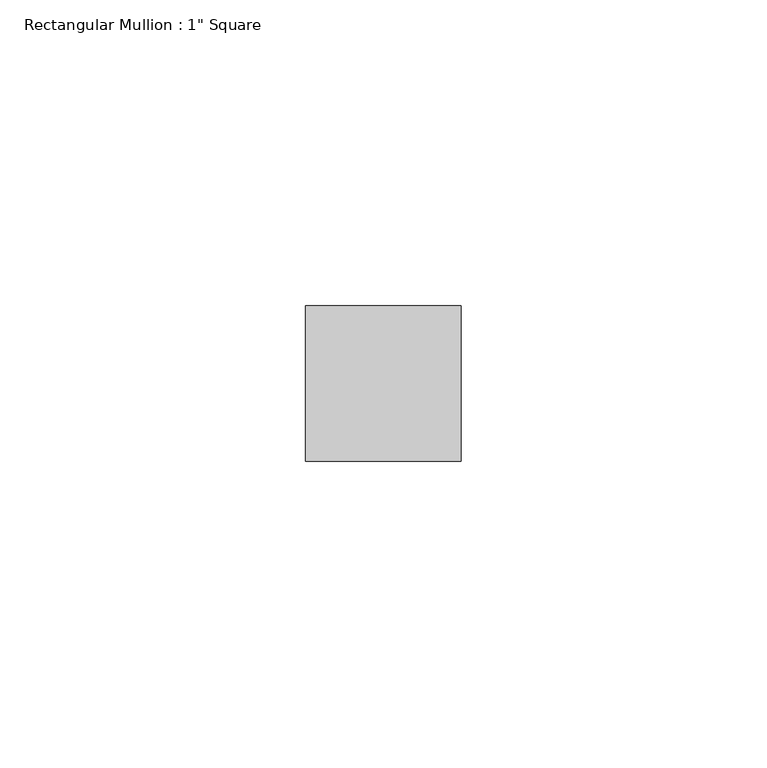
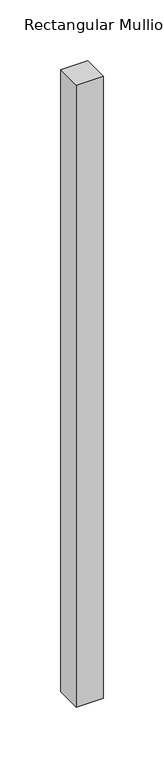
"""IFC4 building model written with IfcOpenShell, lengths in millimetres: member geometry."""

from ifc_helpers import new_model, si_unit, frame, origin, place, context, project, spatial, polyline, outline, extrude, source, transform, mapped, element, save


def member_da69684a(model_context):
    return source(origin(), model_context, "Body", "SweptSolid", [
        extrude(outline(polyline([(12.7, 12.7), (12.7, -12.7), (-12.7, -12.7), (-12.7, 12.7), (12.7, 12.7)])), frame((0.0, 0.0, -624.164422), z_axis=(0.0, 0.0, 1.0), x_axis=(1.0, 0.0, 0.0)), (0.0, 0.0, 1.0), 624.164422),
    ])


if __name__ == "__main__":
    model = new_model("IFC4")
    model_context = context("Model", 3, world=origin())
    ifc_project = project(units=[si_unit("LENGTHUNIT", "METRE", prefix="MILLI")], contexts=[model_context])
    site = spatial("IfcSite", under=ifc_project)
    building = spatial("IfcBuilding", under=site)
    placement = place(None, origin())
    member_shape = member_da69684a(model_context)
    element("IfcMember", 1, ObjectType="Rectangular Mullion : 1\" Square", at=placement, inside=building, context=model_context, shape_type="MappedRepresentation", body=[
        mapped(member_shape, transform((0.0, 0.0, 0.0), x_axis=(1.0, 0.0, 0.0), y_axis=(0.0, 1.0, 0.0), z_axis=(0.0, 0.0, 1.0))),
    ])
    save(model, "model.ifc")

# Revit data of these elements
# Type "Rectangular Mullion : 1\" Square"
#   built-in parameter 1007304 = 0.0833333 (stored number, unit not read)
#   built-in parameter 1007301 = 0.0416667 (stored number, unit not read)
#   built-in parameter 1007300 = 0.0416667 (stored number, unit not read)
# Element 1 (IfcMember, "Rectangular Mullion : 1\" Square")
#   Materials on its faces: "Metal - Aluminum"
# Materials
#   "Metal - Aluminum": class "Metal", colour RGB 247 247 247, transparency 0
